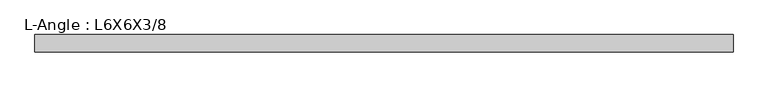
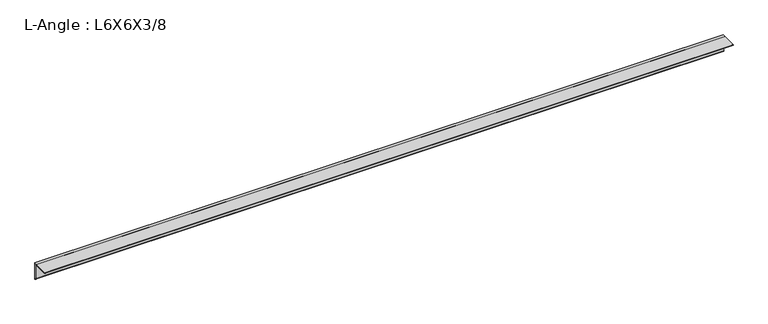
"""IFC4 building model written with IfcOpenShell, lengths in millimetres: member geometry, L-Angle : L6X6X3/8."""

from ifc_helpers import new_model, si_unit, point, frame, frame_2d, origin, place, context, project, spatial, polyline, circle_curve, trimmed, segment, composite_curve, outline, extrude, source, transform, mapped, element, save


def l_angle_l6x6x3_8_2b984bf3(model_context):
    return source(origin(), model_context, "Body", "SweptSolid", [
        extrude(outline(composite_curve([segment(polyline([(41.148, 41.148), (41.148, -111.252)]), True, "CONTINUOUS"), segment(trimmed(circle_curve(frame_2d((41.148, -101.727)), 9.525), [point((41.148, -111.252))], [point((31.623, -101.727))], False, "CARTESIAN"), True, "CONTINUOUS"), segment(polyline([(31.623, -101.727), (31.623, 22.098)]), True, "CONTINUOUS"), segment(trimmed(circle_curve(frame_2d((22.098, 22.098)), 9.525), [point((31.623, 22.098))], [point((22.098, 31.623))], True, "CARTESIAN"), True, "CONTINUOUS"), segment(polyline([(22.098, 31.623), (-101.727, 31.623)]), True, "CONTINUOUS"), segment(trimmed(circle_curve(frame_2d((-101.727, 41.148)), 9.525), [point((-101.727, 31.623))], [point((-111.252, 41.148))], False, "CARTESIAN"), True, "CONTINUOUS"), segment(polyline([(-111.252, 41.148), (41.148, 41.148)]), True, "CONTINUOUS")], self_intersect=False)), frame((-3088.1296112, 0.0, 0.0), z_axis=(1.0, 0.0, 0.0), x_axis=(0.0, 1.0, 0.0)), (0.0, 0.0, 1.0), 6142.746295),
    ])


if __name__ == "__main__":
    model = new_model("IFC4")
    model_context = context("Model", 3, world=origin())
    ifc_project = project(units=[si_unit("LENGTHUNIT", "METRE", prefix="MILLI")], contexts=[model_context])
    site = spatial("IfcSite", under=ifc_project)
    building = spatial("IfcBuilding", under=site)
    placement = place(None, origin())
    l_angle_l6x6x3_8_shape = l_angle_l6x6x3_8_2b984bf3(model_context)
    element("IfcMember", 1, ObjectType="L-Angle : L6X6X3/8", at=placement, inside=building, context=model_context, shape_type="MappedRepresentation", body=[
        mapped(l_angle_l6x6x3_8_shape, transform((0.0, 0.0, 0.0), x_axis=(1.0, 0.0, 0.0), y_axis=(0.0, 1.0, 0.0), z_axis=(0.0, 0.0, 1.0))),
    ])
    save(model, "model.ifc")

# Revit data of these elements
# Type "L-Angle : L6X6X3/8"
#   Assembly Code = "B10"
#   k = 0' - 0 7/8"
#   W = 14.9
#   Length [instance default] = 5' - 0"
#   b = 0' - 6"
#   d = 0' - 6"
#   t = 0' - 0 3/8"
#   x = 0' - 1.62"
#   y = 0' - 1.62"
#   A = 0.0304167 SF
#   Structural Material [instance default] = Steel ASTM A36
# Element 1 (IfcMember, "L-Angle : L6X6X3/8")
#   Materials on its faces: "Steel ASTM A36"
# Materials
#   "Steel ASTM A36": class "Metal", colour RGB 199 199 199, transparency 0, Description = "Structural steel, ASTM A36 Grade B, mill finish", Cost = 0
